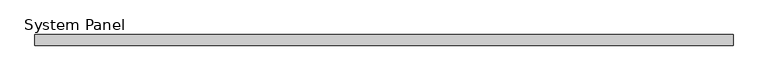
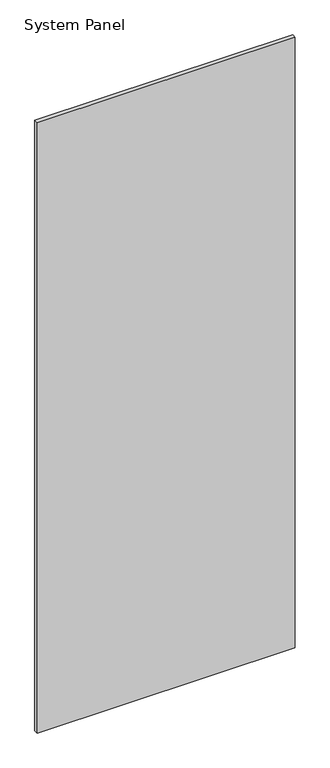
"""IFC4 building model written with IfcOpenShell, lengths in millimetres: plate geometry, System Panel : WWm-Glass-20mm-10mmOffset."""

from ifc_helpers import new_model, si_unit, origin, origin_with_axes, place, context, project, spatial, polyline, outline, extrude, source, transform, mapped, element, save


def system_panel_0ade5c51(model_context):
    return source(origin(), model_context, "Body", "SweptSolid", [
        extrude(outline(polyline([(630.0, 0.0), (-630.0, 0.0), (-630.0, 20.0), (630.0, 20.0), (630.0, 0.0)])), origin_with_axes(), (0.0, 0.0, 1.0), 3150.0),
    ])


if __name__ == "__main__":
    model = new_model("IFC4")
    model_context = context("Model", 3, world=origin())
    ifc_project = project(units=[si_unit("LENGTHUNIT", "METRE", prefix="MILLI")], contexts=[model_context])
    site = spatial("IfcSite", under=ifc_project)
    building = spatial("IfcBuilding", under=site)
    placement = place(None, origin())
    system_panel_shape = system_panel_0ade5c51(model_context)
    element("IfcPlate", 1, ObjectType="System Panel : WWm-Glass-20mm-10mmOffset", at=placement, inside=building, context=model_context, shape_type="MappedRepresentation", body=[
        mapped(system_panel_shape, transform((0.0, 0.0, 0.0), x_axis=(1.0, 0.0, 0.0), y_axis=(0.0, 1.0, 0.0), z_axis=(0.0, 0.0, 1.0))),
    ])
    save(model, "model.ifc")

# Revit data of these elements
# Type "System Panel : WWm-Glass-20mm-10mmOffset"
#   Finish = ""
# Element 1 (IfcPlate, "System Panel : WWm-Glass-20mm-10mmOffset")
#   Materials on its faces: "WW-EC-GL-Storefront"
# Materials
#   "WW-EC-GL-Storefront": class "Glass", colour RGB 236 240 239, transparency 0.85, Description = "Storefront Glass", Cost = 0
